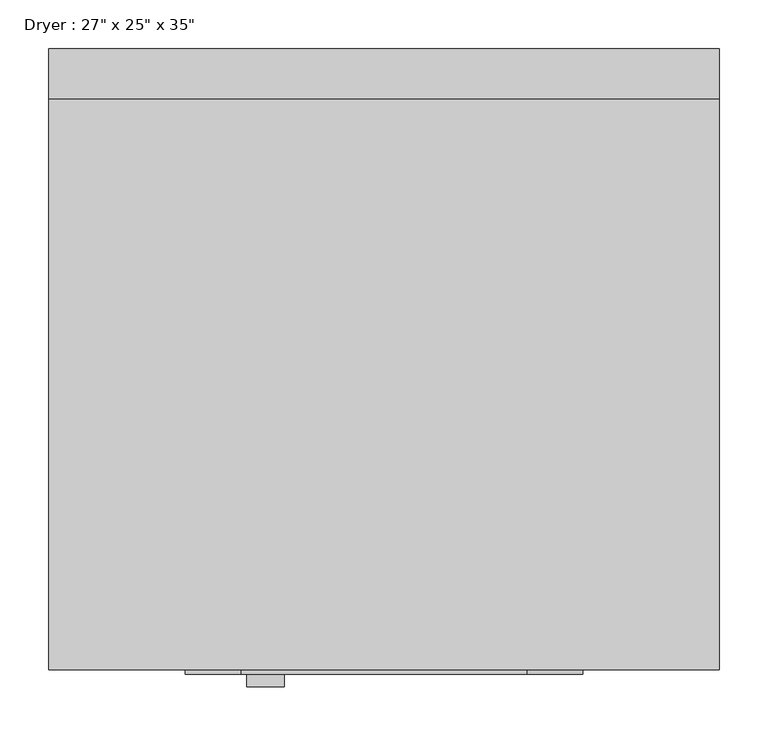
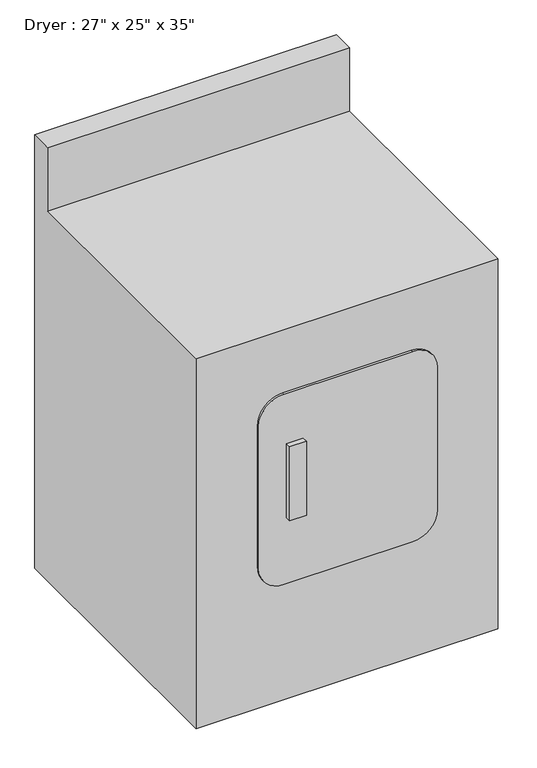
"""IFC4 building model written with IfcOpenShell, lengths in millimetres: proxy geometry."""

import ifcopenshell
import ifcopenshell.guid

model = None  # the IFC model being written
_history = None  # IfcOwnerHistory: only IFC2X3 demands one
_inside = {}  # id of a spatial element -> (the spatial element, [elements in it])
_under = {}  # id of a project, library or spatial element -> (it, [spatial elements below it])
_declared = {}  # id of a project -> (the project, [libraries it declares])
_typed = {}  # id of a type object -> (the type object, [elements of that type])
_made_of = {}  # id of a material, layer set ... -> (it, [elements and type objects made of it])


def new_model(schema):
    """Start an empty IFC model of exactly this schema.

    Asked for "IFC4X3", IfcOpenShell would pick the latest addendum, in which some entities
    have other attributes; the version numbers below select the first issue.
    IFC2X3 requires an IfcOwnerHistory on every rooted entity: one is made here for all.
    """
    global model, _history
    if schema == "IFC4X3":
        model = ifcopenshell.file(schema_version=(4, 3, 0, 0))
    else:
        model = ifcopenshell.file(schema=schema)
    _inside.clear()
    _under.clear()
    _declared.clear()
    _typed.clear()
    _made_of.clear()
    _history = None
    if model.schema == "IFC2X3":
        org = make("IfcOrganization", Name="unknown")
        user = make(
            "IfcPersonAndOrganization",
            ThePerson=make("IfcPerson", FamilyName="unknown"),
            TheOrganization=org,
        )
        app = make(
            "IfcApplication",
            ApplicationDeveloper=org,
            Version="unknown",
            ApplicationFullName="unknown",
            ApplicationIdentifier="unknown",
        )
        _history = make(
            "IfcOwnerHistory",
            OwningUser=user,
            OwningApplication=app,
            ChangeAction="ADDED",
            CreationDate=0,
        )
    return model


def make(cls, **values):
    """One entity of the class cls with the attributes given. An attribute that is None is left unset."""
    return model.create_entity(
        cls, **{name: value for name, value in values.items() if value is not None}
    )


def rooted(cls, **values):
    """An entity with a GlobalId (a new one), such as an element, a storey or a relation."""
    return make(cls, GlobalId=ifcopenshell.guid.new(), OwnerHistory=_history, **values)


def si_unit(unit_type, name, prefix=None):
    """IfcSIUnit, for example si_unit("LENGTHUNIT", "METRE", prefix="MILLI")."""
    return make("IfcSIUnit", UnitType=unit_type, Prefix=prefix, Name=name)


def assignment(units):
    """IfcUnitAssignment: the units of a project."""
    return None if units is None else make("IfcUnitAssignment", Units=units)


def point(xyz):
    """IfcCartesianPoint."""
    return None if xyz is None else make("IfcCartesianPoint", Coordinates=xyz)


def direction(xyz):
    """IfcDirection."""
    return None if xyz is None else make("IfcDirection", DirectionRatios=xyz)


def frame(location, z_axis=None, x_axis=None):
    """IfcAxis2Placement3D, a coordinate frame: its origin and axes. An axis left out is left unset."""
    return make(
        "IfcAxis2Placement3D",
        Location=point(location),
        Axis=direction(z_axis),
        RefDirection=direction(x_axis),
    )


def frame_2d(location, x_axis=None):
    """IfcAxis2Placement2D, a coordinate frame in the plane: its origin and x axis."""
    return make(
        "IfcAxis2Placement2D", Location=point(location), RefDirection=direction(x_axis)
    )


def origin():
    """The frame at (0, 0, 0) with its axes left unset."""
    return frame((0.0, 0.0, 0.0))


def place(relative_to, where):
    """IfcLocalPlacement: puts the frame where relative to a parent placement (None: the world)."""
    return make(
        "IfcLocalPlacement", PlacementRelTo=relative_to, RelativePlacement=where
    )


def context(
    kind, dimensions, precision=None, world=None, true_north=None, identifier=None
):
    """IfcGeometricRepresentationContext, for example the 3D "Model" context."""
    return make(
        "IfcGeometricRepresentationContext",
        ContextIdentifier=identifier,
        ContextType=kind,
        CoordinateSpaceDimension=dimensions,
        Precision=precision,
        WorldCoordinateSystem=world,
        TrueNorth=true_north,
    )


def project(units=None, contexts=None):
    """IfcProject with its units and contexts."""
    return rooted(
        "IfcProject",
        Name="project",
        RepresentationContexts=contexts,
        UnitsInContext=assignment(units),
    )


def spatial(cls, under=None, at=None, **own):
    """A site, building, storey or space (cls), placed at a placement, below another one or the project."""
    s = rooted(cls, ObjectPlacement=at, **own)
    if under is not None:
        _under.setdefault(under.id(), (under, []))[1].append(s)
    return s


def polyline(points):
    """IfcPolyline through the points."""
    return make("IfcPolyline", Points=[point(p) for p in points])


def circle_curve(where, radius):
    """IfcCircle in the frame where."""
    return make("IfcCircle", Position=where, Radius=radius)


def trimmed(basis, trim1, trim2, sense, master):
    """IfcTrimmedCurve: the piece of a basis curve between two trims."""
    return make(
        "IfcTrimmedCurve",
        BasisCurve=basis,
        Trim1=trim1,
        Trim2=trim2,
        SenseAgreement=sense,
        MasterRepresentation=master,
    )


def segment(curve, same_sense, transition):
    """IfcCompositeCurveSegment."""
    return make(
        "IfcCompositeCurveSegment",
        Transition=transition,
        SameSense=same_sense,
        ParentCurve=curve,
    )


def composite_curve(segments, self_intersect=None):
    """IfcCompositeCurve: segments joined end to end."""
    return make("IfcCompositeCurve", Segments=segments, SelfIntersect=self_intersect)


def outline(outer, holes=None, kind="AREA"):
    """IfcArbitraryClosedProfileDef: a profile drawn as a closed curve; with holes, ...WithVoids."""
    if holes is None:
        return make("IfcArbitraryClosedProfileDef", ProfileType=kind, OuterCurve=outer)
    return make(
        "IfcArbitraryProfileDefWithVoids",
        ProfileType=kind,
        OuterCurve=outer,
        InnerCurves=holes,
    )


def extrude(swept, where, along, depth):
    """IfcExtrudedAreaSolid: the profile swept, set in the frame where, extruded along a direction by depth."""
    return make(
        "IfcExtrudedAreaSolid",
        SweptArea=swept,
        Position=where,
        ExtrudedDirection=direction(along),
        Depth=depth,
    )


def shape(context_of_items, identifier, shape_type, items):
    """IfcShapeRepresentation: the items that make up one representation, for example the "Body"."""
    return make(
        "IfcShapeRepresentation",
        ContextOfItems=context_of_items,
        RepresentationIdentifier=identifier,
        RepresentationType=shape_type,
        Items=items,
    )


def source(mapping_origin, context_of_items, identifier, shape_type, items):
    """IfcRepresentationMap: a shape defined once, which mapped items show again and again."""
    return make(
        "IfcRepresentationMap",
        MappingOrigin=mapping_origin,
        MappedRepresentation=shape(context_of_items, identifier, shape_type, items),
    )


def transform(
    local_origin,
    x_axis=None,
    y_axis=None,
    z_axis=None,
    scale=None,
    scale2=None,
    scale3=None,
    uniform=True,
):
    """IfcCartesianTransformationOperator3D, or its non-uniform kind. x_axis, y_axis, z_axis: its Axis1, 2, 3."""
    if uniform:
        return make(
            "IfcCartesianTransformationOperator3D",
            Axis1=direction(x_axis),
            Axis2=direction(y_axis),
            LocalOrigin=point(local_origin),
            Scale=scale,
            Axis3=direction(z_axis),
        )
    return make(
        "IfcCartesianTransformationOperator3DnonUniform",
        Axis1=direction(x_axis),
        Axis2=direction(y_axis),
        LocalOrigin=point(local_origin),
        Scale=scale,
        Axis3=direction(z_axis),
        Scale2=scale2,
        Scale3=scale3,
    )


def mapped(mapping_source, mapping_target):
    """IfcMappedItem: shows the shape of a source again, moved by a transform."""
    return make(
        "IfcMappedItem", MappingSource=mapping_source, MappingTarget=mapping_target
    )


def made_of(thing, what):
    """Note that an element or type object is made of a material, layer set ...; save() writes the relation."""
    if what is not None:
        _made_of.setdefault(what.id(), (what, []))[1].append(thing)
    return thing


def element(
    cls,
    number,
    at=None,
    inside=None,
    cuts=None,
    type_object=None,
    material=None,
    context=None,
    identifier="Body",
    shape_type=None,
    held_by="IfcProductDefinitionShape",
    body=None,
    shapes=None,
    **own,
):
    """One element of the class cls, such as IfcWall. Its Tag is "e" and its number.

    at: its placement. inside: the storey or other place that contains it. cuts: it is an
    opening in that element (IfcRelVoidsElement). A single representation is given by context,
    identifier, shape_type and body (its items); several are given by shapes. held_by: the class
    of the entity that holds the representations. save() writes the other relations.
    """
    e = rooted(cls, Tag="e%d" % number, ObjectPlacement=at, **own)
    if body is not None:
        shapes = [shape(context, identifier, shape_type, body)]
    if shapes is not None:
        e.Representation = make(held_by, Representations=shapes)
    if inside is not None:
        _inside.setdefault(inside.id(), (inside, []))[1].append(e)
    if cuts is not None:
        rooted(
            "IfcRelVoidsElement", RelatingBuildingElement=cuts, RelatedOpeningElement=e
        )
    if type_object is not None:
        _typed.setdefault(type_object.id(), (type_object, []))[1].append(e)
    return made_of(e, material)


def aggregate(whole, parts):
    """IfcRelAggregates: a whole, such as a stair, and the parts it consists of."""
    return rooted("IfcRelAggregates", RelatingObject=whole, RelatedObjects=parts)


def save(model, path):
    """Write the relations noted so far, then the file.

    IfcRelAggregates (storeys below a building ...), IfcRelContainedInSpatialStructure (elements
    in a storey), IfcRelDefinesByType, IfcRelAssociatesMaterial and IfcRelDeclares: one each for
    every whole, place, type object, material and project.
    """
    for whole, parts in _under.values():
        aggregate(whole, parts)
    for where, things in _inside.values():
        rooted(
            "IfcRelContainedInSpatialStructure",
            RelatedElements=things,
            RelatingStructure=where,
        )
    for kind, things in _typed.values():
        rooted("IfcRelDefinesByType", RelatedObjects=things, RelatingType=kind)
    for what, things in _made_of.values():
        rooted("IfcRelAssociatesMaterial", RelatedObjects=things, RelatingMaterial=what)
    for by, libraries in _declared.values():
        rooted("IfcRelDeclares", RelatingContext=by, RelatedDefinitions=libraries)
    model.write(path)


def proxy_b4d0e45e(model_context):
    return source(origin(), model_context, "Body", "SweptSolid", [
        extrude(outline(polyline([(276.7635206, -20.3014962), (238.6635206, -20.3014962), (238.6635206, -7.6014962), (276.7635206, -7.6014962), (276.7635206, -20.3014962)])), frame((0.0, 0.0, 438.7649313), z_axis=(0.0, 0.0, 1.0), x_axis=(1.0, 0.0, 0.0)), (0.0, 0.0, 1.0), 177.8),
        extrude(outline(composite_curve([segment(polyline([(737.623844, 525.0374563), (737.623844, 232.9374563)]), True, "CONTINUOUS"), segment(trimmed(circle_curve(frame_2d((680.473844, 232.9374563)), 57.15), [point((737.623844, 232.9374563))], [point((680.473844, 175.7874563))], False, "CARTESIAN"), True, "CONTINUOUS"), segment(polyline([(680.473844, 175.7874563), (337.573844, 175.7874563)]), True, "CONTINUOUS"), segment(trimmed(circle_curve(frame_2d((337.573844, 232.9374563)), 57.15), [point((337.573844, 175.7874563))], [point((280.423844, 232.9374563))], False, "CARTESIAN"), True, "CONTINUOUS"), segment(polyline([(280.423844, 232.9374563), (280.423844, 525.0374563)]), True, "CONTINUOUS"), segment(trimmed(circle_curve(frame_2d((337.573844, 525.0374563)), 57.15), [point((280.423844, 525.0374563))], [point((337.573844, 582.1874563))], False, "CARTESIAN"), True, "CONTINUOUS"), segment(polyline([(337.573844, 582.1874563), (680.473844, 582.1874563)]), True, "CONTINUOUS"), segment(trimmed(circle_curve(frame_2d((680.473844, 525.0374563)), 57.15), [point((680.473844, 582.1874563))], [point((737.623844, 525.0374563))], False, "CARTESIAN"), True, "CONTINUOUS")], self_intersect=False)), frame((0.0, -7.6014962, 0.0), z_axis=(0.0, 1.0, 0.0), x_axis=(0.0, 0.0, 1.0)), (0.0, 0.0, 1.0), 4.7625),
        extrude(outline(polyline([(632.1610038, 0.0), (-2.8389962, 0.0), (-2.8389962, 889.0), (581.3610038, 889.0), (581.3610038, 1041.4), (632.1610038, 1041.4), (632.1610038, 0.0)])), frame((36.0874563, 0.0, 0.0), z_axis=(1.0, 0.0, 0.0), x_axis=(0.0, 1.0, 0.0)), (0.0, 0.0, 1.0), 685.8),
    ])


if __name__ == "__main__":
    model = new_model("IFC4")
    model_context = context("Model", 3, world=origin())
    ifc_project = project(units=[si_unit("LENGTHUNIT", "METRE", prefix="MILLI")], contexts=[model_context])
    site = spatial("IfcSite", under=ifc_project)
    building = spatial("IfcBuilding", under=site)
    placement = place(None, origin())
    proxy_shape = proxy_b4d0e45e(model_context)
    element("IfcBuildingElementProxy", 1, Name="Dryer : 27\" x 25\" x 35\"", ObjectType="Dryer : 27\" x 25\" x 35\"", at=placement, inside=building, context=model_context, shape_type="MappedRepresentation", body=[
        mapped(proxy_shape, transform((0.0, 0.0, 0.0), x_axis=(1.0, 0.0, 0.0), y_axis=(0.0, 1.0, 0.0), z_axis=(0.0, 0.0, 1.0))),
    ])
    save(model, "model.ifc")

# Revit data of these elements
# Type "Dryer : 27\" x 25\" x 35\""
#   Label = "D"
#   Assembly Code = "E1090400"
#   Depth = 2' - 1"
#   Height = 2' - 11"
#   Width = 2' - 3"
#   Dryer Material = Metal - Paint Finish - Ivory, Glossy
# Element 1 (IfcBuildingElementProxy, "Dryer : 27\" x 25\" x 35\"")
#   Materials on its faces: "Metal - Paint Finish - Ivory, Glossy"
# Materials
#   "Metal - Paint Finish - Ivory, Glossy": class "Paint", colour RGB 247 247 239, transparency 0
